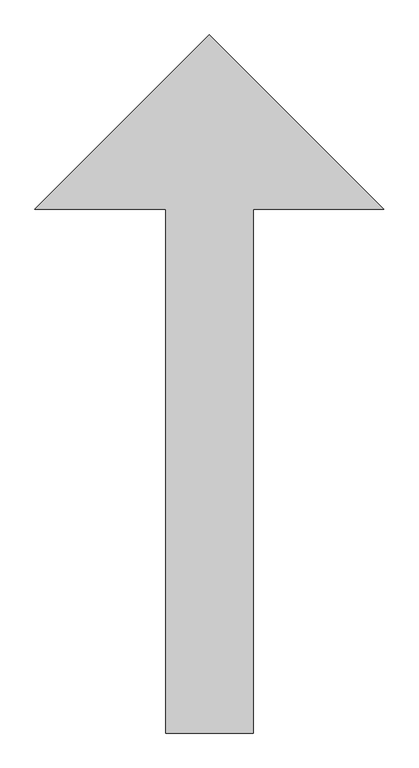
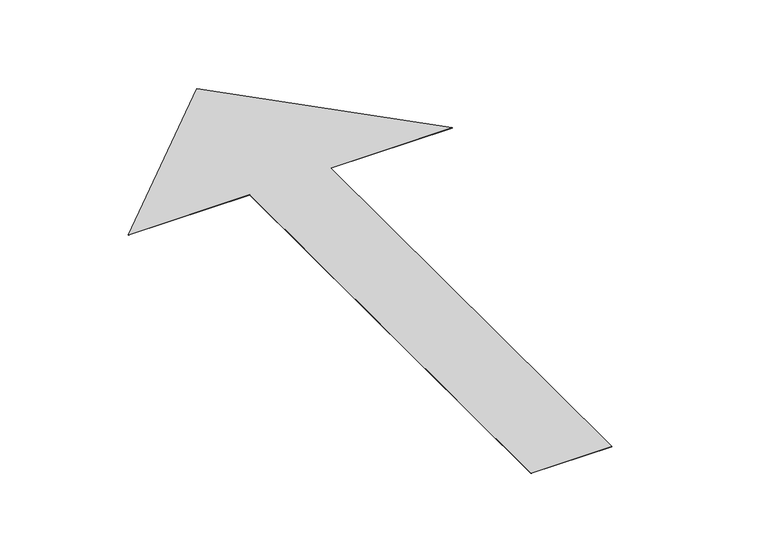
"""IFC4 building model written with IfcOpenShell, lengths in millimetres: proxy geometry, NLRS_90_PA_LB_pijl bewegwijzering_gen_rsf : pijl bewegwijzering."""

from ifc_helpers import new_model, si_unit, origin, origin_with_axes, place, context, project, spatial, polyline, outline, extrude, source, transform, mapped, element, save


def parking_0bd23258(model_context):
    return source(origin(), model_context, "Body", "SweptSolid", [
        extrude(outline(polyline([(-125.0, 0.0), (375.0, -500.0), (0.0, -500.0), (0.0, -2000.0), (-250.0, -2000.0), (-250.0, -500.0), (-625.0, -500.0), (-125.0, 0.0)])), origin_with_axes(), (0.0, 0.0, 1.0), 1.0),
    ])


if __name__ == "__main__":
    model = new_model("IFC4")
    model_context = context("Model", 3, world=origin())
    ifc_project = project(units=[si_unit("LENGTHUNIT", "METRE", prefix="MILLI")], contexts=[model_context])
    site = spatial("IfcSite", under=ifc_project)
    building = spatial("IfcBuilding", under=site)
    placement = place(None, origin())
    parking_shape = parking_0bd23258(model_context)
    element("IfcBuildingElementProxy", 1, Name="NLRS_90_PA_LB_pijl bewegwijzering_gen_rsf : pijl bewegwijzering", ObjectType="NLRS_90_PA_LB_pijl bewegwijzering_gen_rsf : pijl bewegwijzering", at=placement, inside=building, context=model_context, shape_type="MappedRepresentation", body=[
        mapped(parking_shape, transform((0.0, 0.0, 0.0), x_axis=(1.0, 0.0, 0.0), y_axis=(0.0, 1.0, 0.0), z_axis=(0.0, 0.0, 1.0))),
    ])
    save(model, "model.ifc")

# Revit data of these elements
# Type "NLRS_90_PA_LB_pijl bewegwijzering_gen_rsf : pijl bewegwijzering"
#   Type IFC Predefined Type = "USERDEFINED"
#   Export Type to IFC As = "IfcBuildingElementProxyType"
#   Type IfcGUID = "2C9lkgojj1sel6c4s_vQ2Q"
#   IfcName[Type] = "pijl bewegwijzering"
#   IfcDescription[Type] = "pijl bewegwijzering"
#   IfcObjectType[Type] = "SIGNAGE"
#   IfcExportAs[Type] = "IfcBuildingElementProxyType"
#   IfcExportType[Type] = "USERDEFINED"
#   Description = "pijl bewegwijzering"
#   Assembly Code = "90.72"
#   Pijlbreedte = 250.00 mm
#   Lengte_pijl = 2000.00 mm
#   Dikte_belijning = 1.00 mm
#   Materiaal_belijning = NLRS_v4_verf ivoorkleurig mat_gen_rsf
# Element 1 (IfcBuildingElementProxy, "NLRS_90_PA_LB_pijl bewegwijzering_gen_rsf : pijl bewegwijzering")
#   Materials on its faces: "NLRS_v4_verf ivoorkleurig mat_gen_rsf"
# Materials
#   "NLRS_v4_verf ivoorkleurig mat_gen_rsf": class "V - Verven", colour RGB 216 216 204, transparency 0, Keynote = "v4", Manufacturer = "Revit Standards Foundation", URL = "www.revitstandards.org", Description = "verf ivoorkleurig mat", Cost = 0
